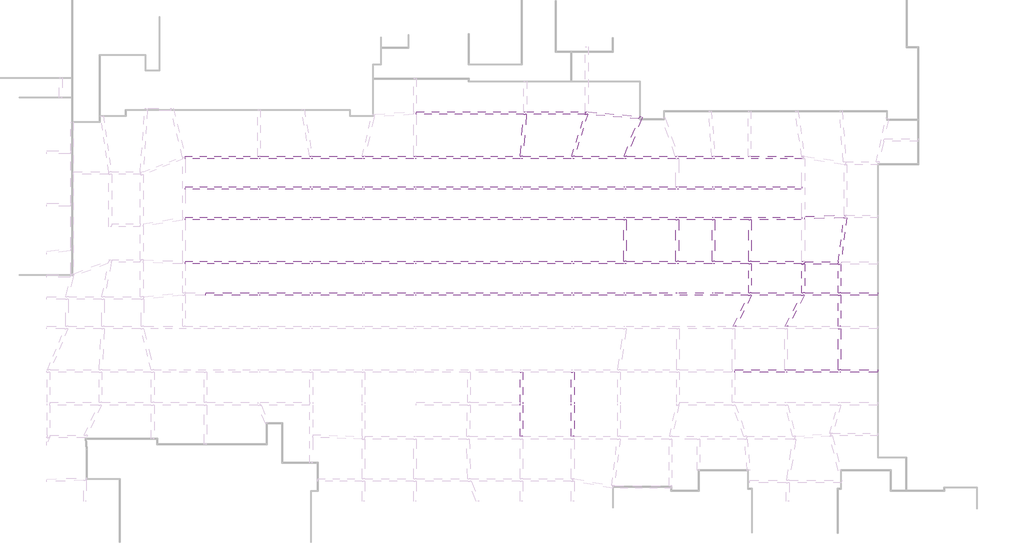
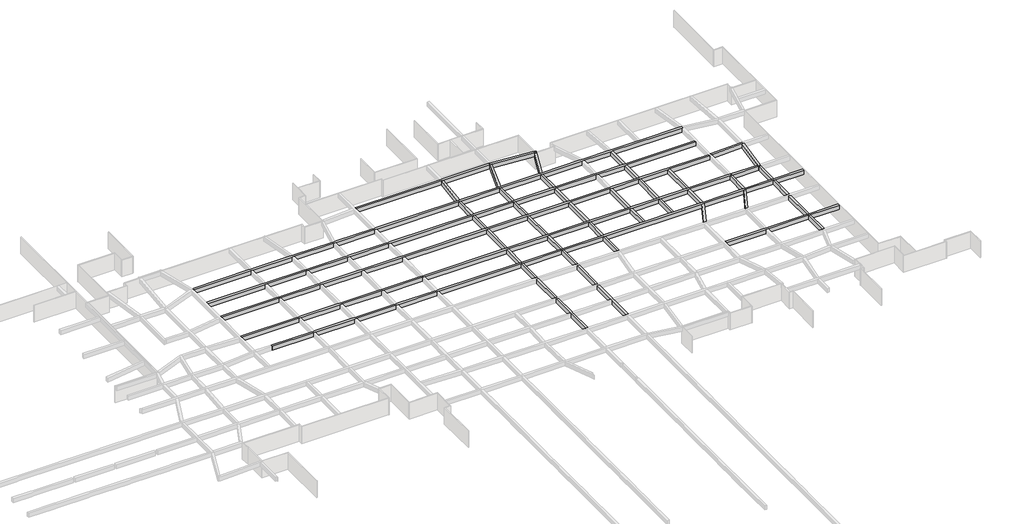
# One storey, part 44 of 45: 27 beams.
"""IFC4 building model written with IfcOpenShell, lengths in millimetres."""

from ifc_helpers import new_model, si_unit, frame, origin, place, context, project, spatial, polyline, outline, extrude, faceted_brep, element, save

model = new_model("IFC4")

# Units and contexts
model_context = context("Model", 3, world=origin())
ifc_project = project(units=[si_unit("LENGTHUNIT", "METRE", prefix="MILLI")], contexts=[model_context])

# Site, building, storey
site = spatial("IfcSite", under=ifc_project)
building = spatial("IfcBuilding", under=site)
storey = spatial("IfcBuildingStorey", under=building, Name="户型图", Elevation=0.0)

# Beams
placement = place(None, origin())
element("IfcBeam", 1, ObjectType="混凝土 - 矩形梁 : KL_beam", at=placement, inside=storey, context=model_context, shape_type="Brep", body=[
    faceted_brep([(63459.0283671, 163994.6607145, 3300.0), (63459.0283671, 163594.6607145, 3300.0), (63459.0283671, 163594.6607145, 2500.0), (63459.0283671, 163994.6607145, 2500.0), (57931.1254195, 163994.6607145, 3300.0), (57531.1254195, 163994.6607145, 3300.0), (52492.4652495, 163994.6607145, 3300.0), (52092.4652495, 163994.6607145, 3300.0), (44558.170888, 163994.6607145, 3300.0), (44158.170888, 163994.6607145, 3300.0), (39058.170888, 163994.6607145, 3300.0), (38658.170888, 163994.6607145, 3300.0), (33658.170888, 163994.6607145, 3300.0), (33258.170888, 163994.6607145, 3300.0), (25858.170888, 163994.6607145, 3300.0), (25458.170888, 163994.6607145, 3300.0), (18058.170888, 163994.6607145, 3300.0), (17658.170888, 163994.6607145, 3300.0), (10373.3027926, 163994.6607145, 3300.0), (9973.3027926, 163994.6607145, 3300.0), (-5504.3123934, 163994.6607145, 3300.0), (-5904.3123934, 163994.6607145, 3300.0), (-13220.6748317, 163994.6607145, 3300.0), (-13620.6748317, 163994.6607145, 3300.0), (-21020.6748317, 163994.6607145, 3300.0), (-21420.6748317, 163994.6607145, 3300.0), (-28820.6748317, 163994.6607145, 3300.0), (-29220.6748317, 163994.6607145, 3300.0), (-37009.4216094, 163994.6607145, 3300.0), (-37009.4216094, 163994.4687414, 3300.0), (-37009.4216094, 163594.6607145, 3300.0), (-29220.6748317, 163594.6607145, 3300.0), (-28820.6748317, 163594.6607145, 3300.0), (-21420.6748317, 163594.6607145, 3300.0), (-21020.6748317, 163594.6607145, 3300.0), (-13620.6748317, 163594.6607145, 3300.0), (-13220.6748317, 163594.6607145, 3300.0), (-5904.3123934, 163594.6607145, 3300.0), (-5504.3123934, 163594.6607145, 3300.0), (9973.3027926, 163594.6607145, 3300.0), (10373.3027926, 163594.6607145, 3300.0), (17658.170888, 163594.6607145, 3300.0), (18058.170888, 163594.6607145, 3300.0), (25458.170888, 163594.6607145, 3300.0), (25858.170888, 163594.6607145, 3300.0), (44084.7377305, 163594.6607145, 3300.0), (44529.7785067, 163594.6607145, 3300.0), (51966.0949121, 163594.6607145, 3300.0), (52415.0254072, 163594.6607145, 3300.0), (57531.1254195, 163594.6607145, 3300.0), (57931.1254195, 163594.6607145, 3300.0), (-37009.4216094, 163594.6607145, 2500.0), (-29220.6748317, 163594.6607145, 2500.0), (-28820.6748317, 163594.6607145, 2500.0), (-21420.6748317, 163594.6607145, 2500.0), (-21020.6748317, 163594.6607145, 2500.0), (-13620.6748317, 163594.6607145, 2500.0), (-13220.6748317, 163594.6607145, 2500.0), (-5904.3123934, 163594.6607145, 2500.0), (-5504.3123934, 163594.6607145, 2500.0), (9973.3027926, 163594.6607145, 2500.0), (10373.3027926, 163594.6607145, 2500.0), (17658.170888, 163594.6607145, 2500.0), (18058.170888, 163594.6607145, 2500.0), (25458.170888, 163594.6607145, 2500.0), (25858.170888, 163594.6607145, 2500.0), (44084.7377305, 163594.6607145, 2500.0), (44529.7785067, 163594.6607145, 2500.0), (51966.0949121, 163594.6607145, 2500.0), (52415.0254072, 163594.6607145, 2500.0), (57531.1254195, 163594.6607145, 2500.0), (57931.1254195, 163594.6607145, 2500.0), (-37009.4216094, 163994.4687414, 2500.0), (-37009.4216094, 163994.6607145, 2500.0), (-29220.6748317, 163994.6607145, 2500.0), (-28820.6748317, 163994.6607145, 2500.0), (-21420.6748317, 163994.6607145, 2500.0), (-21020.6748317, 163994.6607145, 2500.0), (-13620.6748317, 163994.6607145, 2500.0), (-13220.6748317, 163994.6607145, 2500.0), (-5904.3123934, 163994.6607145, 2500.0), (-5504.3123934, 163994.6607145, 2500.0), (9973.3027926, 163994.6607145, 2500.0), (10373.3027926, 163994.6607145, 2500.0), (17658.170888, 163994.6607145, 2500.0), (18058.170888, 163994.6607145, 2500.0), (25458.170888, 163994.6607145, 2500.0), (25858.170888, 163994.6607145, 2500.0), (33258.170888, 163994.6607145, 2500.0), (33658.170888, 163994.6607145, 2500.0), (38658.170888, 163994.6607145, 2500.0), (39058.170888, 163994.6607145, 2500.0), (44158.170888, 163994.6607145, 2500.0), (44558.170888, 163994.6607145, 2500.0), (52092.4652495, 163994.6607145, 2500.0), (52492.4652495, 163994.6607145, 2500.0), (57531.1254195, 163994.6607145, 2500.0), (57931.1254195, 163994.6607145, 2500.0)], [[[0, 1, 2, 3]], [[1, 0, 4, 5, 6, 7, 8, 9, 10, 11, 12, 13, 14, 15, 16, 17, 18, 19, 20, 21, 22, 23, 24, 25, 26, 27, 28, 29, 30, 31, 32, 33, 34, 35, 36, 37, 38, 39, 40, 41, 42, 43, 44, 45, 46, 47, 48, 49, 50]], [[2, 1, 50, 49, 48, 47, 46, 45, 44, 43, 42, 41, 40, 39, 38, 37, 36, 35, 34, 33, 32, 31, 30, 51, 52, 53, 54, 55, 56, 57, 58, 59, 60, 61, 62, 63, 64, 65, 66, 67, 68, 69, 70, 71]], [[3, 2, 71, 70, 69, 68, 67, 66, 65, 64, 63, 62, 61, 60, 59, 58, 57, 56, 55, 54, 53, 52, 51, 72, 73, 74, 75, 76, 77, 78, 79, 80, 81, 82, 83, 84, 85, 86, 87, 88, 89, 90, 91, 92, 93, 94, 95, 96, 97]], [[0, 3, 97, 96, 95, 94, 93, 92, 91, 90, 89, 88, 87, 86, 85, 84, 83, 82, 81, 80, 79, 78, 77, 76, 75, 74, 73, 28, 27, 26, 25, 24, 23, 22, 21, 20, 19, 18, 17, 16, 15, 14, 13, 12, 11, 10, 9, 8, 7, 6, 5, 4]], [[28, 73, 72, 51, 30, 29]]]),
])
element("IfcBeam", 2, ObjectType="混凝土 - 矩形梁 : KL_beam", at=placement, inside=storey, context=model_context, shape_type="Brep", body=[
    faceted_brep([(52292.9021454, 184394.3140025, 3300.0), (52048.8431015, 184394.3140025, 3300.0), (44458.170888, 184394.3140025, 3300.0), (44058.170888, 184394.3140025, 3300.0), (39044.6739052, 184394.3140025, 3300.0), (38643.697146, 184394.3140025, 3300.0), (33600.8295016, 184394.3140025, 3300.0), (33177.7812291, 184394.3140025, 3300.0), (25952.5239413, 184394.3140025, 3300.0), (25522.3855905, 184394.3140025, 3300.0), (18130.3080686, 184394.3140025, 3300.0), (17711.1861948, 184394.3140025, 3300.0), (10391.598587, 184394.3140025, 3300.0), (9990.070652, 184394.3140025, 3300.0), (-5504.3123934, 184394.3140025, 3300.0), (-5904.3123934, 184394.3140025, 3300.0), (-13169.2403719, 184394.3140025, 3300.0), (-13579.762015, 184394.3140025, 3300.0), (-21052.8549054, 184394.3140025, 3300.0), (-21459.0255502, 184394.3140025, 3300.0), (-28820.6748317, 184394.3140025, 3300.0), (-29220.6748317, 184394.3140025, 3300.0), (-40064.3312613, 184394.3140025, 3300.0), (-40020.6748317, 184219.2176267, 3300.0), (-40020.6748317, 183994.3140025, 3300.0), (-29220.6748317, 183994.3140025, 3300.0), (-28820.6748317, 183994.3140025, 3300.0), (-21420.6748317, 183994.3140025, 3300.0), (-21020.6748317, 183994.3140025, 3300.0), (-13620.6748317, 183994.3140025, 3300.0), (-13220.6748317, 183994.3140025, 3300.0), (-5904.3123934, 183994.3140025, 3300.0), (-5504.3123934, 183994.3140025, 3300.0), (9973.3027926, 183994.3140025, 3300.0), (10373.3027926, 183994.3140025, 3300.0), (17658.170888, 183994.3140025, 3300.0), (18058.170888, 183994.3140025, 3300.0), (25458.170888, 183994.3140025, 3300.0), (25858.170888, 183994.3140025, 3300.0), (33258.170888, 183994.3140025, 3300.0), (33658.170888, 183994.3140025, 3300.0), (38658.170888, 183994.3140025, 3300.0), (39058.170888, 183994.3140025, 3300.0), (52092.6053307, 183994.3140025, 3300.0), (52264.9314206, 183994.3140025, 3300.0), (52264.9314206, 183994.3140025, 2500.0), (-40020.6748317, 183994.3140025, 2500.0), (-29220.6748317, 183994.3140025, 2500.0), (-28820.6748317, 183994.3140025, 2500.0), (-21420.6748317, 183994.3140025, 2500.0), (-21020.6748317, 183994.3140025, 2500.0), (-13620.6748317, 183994.3140025, 2500.0), (-13220.6748317, 183994.3140025, 2500.0), (-5904.3123934, 183994.3140025, 2500.0), (-5504.3123934, 183994.3140025, 2500.0), (9973.3027926, 183994.3140025, 2500.0), (10373.3027926, 183994.3140025, 2500.0), (17658.170888, 183994.3140025, 2500.0), (18058.170888, 183994.3140025, 2500.0), (25458.170888, 183994.3140025, 2500.0), (25858.170888, 183994.3140025, 2500.0), (33258.170888, 183994.3140025, 2500.0), (33658.170888, 183994.3140025, 2500.0), (38658.170888, 183994.3140025, 2500.0), (39058.170888, 183994.3140025, 2500.0), (52092.6053307, 183994.3140025, 2500.0), (-40064.3312613, 184394.3140025, 2500.0), (-29220.6748317, 184394.3140025, 2500.0), (-28820.6748317, 184394.3140025, 2500.0), (-21459.0255502, 184394.3140025, 2500.0), (-21052.8549054, 184394.3140025, 2500.0), (-13579.762015, 184394.3140025, 2500.0), (-13169.2403719, 184394.3140025, 2500.0), (-5904.3123934, 184394.3140025, 2500.0), (-5504.3123934, 184394.3140025, 2500.0), (9990.070652, 184394.3140025, 2500.0), (10391.598587, 184394.3140025, 2500.0), (17711.1861948, 184394.3140025, 2500.0), (18130.3080686, 184394.3140025, 2500.0), (25522.3855905, 184394.3140025, 2500.0), (25952.5239413, 184394.3140025, 2500.0), (33177.7812291, 184394.3140025, 2500.0), (33600.8295016, 184394.3140025, 2500.0), (38643.697146, 184394.3140025, 2500.0), (39044.6739052, 184394.3140025, 2500.0), (44058.170888, 184394.3140025, 2500.0), (44458.170888, 184394.3140025, 2500.0), (52048.8431015, 184394.3140025, 2500.0), (52292.9021454, 184394.3140025, 2500.0), (-40020.6748317, 184219.2176267, 2500.0)], [[[0, 1, 2, 3, 4, 5, 6, 7, 8, 9, 10, 11, 12, 13, 14, 15, 16, 17, 18, 19, 20, 21, 22, 23, 24, 25, 26, 27, 28, 29, 30, 31, 32, 33, 34, 35, 36, 37, 38, 39, 40, 41, 42, 43, 44]], [[45, 44, 43, 42, 41, 40, 39, 38, 37, 36, 35, 34, 33, 32, 31, 30, 29, 28, 27, 26, 25, 24, 46, 47, 48, 49, 50, 51, 52, 53, 54, 55, 56, 57, 58, 59, 60, 61, 62, 63, 64, 65]], [[66, 67, 68, 69, 70, 71, 72, 73, 74, 75, 76, 77, 78, 79, 80, 81, 82, 83, 84, 85, 86, 87, 88, 45, 65, 64, 63, 62, 61, 60, 59, 58, 57, 56, 55, 54, 53, 52, 51, 50, 49, 48, 47, 46, 89]], [[22, 21, 20, 19, 18, 17, 16, 15, 14, 13, 12, 11, 10, 9, 8, 7, 6, 5, 4, 3, 2, 1, 0, 88, 87, 86, 85, 84, 83, 82, 81, 80, 79, 78, 77, 76, 75, 74, 73, 72, 71, 70, 69, 68, 67, 66]], [[89, 23, 22, 66]], [[23, 89, 46, 24]], [[0, 44, 45, 88]]]),
])
element("IfcBeam", 3, ObjectType="混凝土 - 矩形梁 : KL_beam", at=placement, inside=storey, context=model_context, shape_type="Brep", body=[
    faceted_brep([(-40020.6748317, 179811.4368869, 3300.0), (-40020.6748317, 179411.4368869, 3300.0), (-29220.6748317, 179411.4368869, 3300.0), (-28820.6748317, 179411.4368869, 3300.0), (-21420.6748317, 179411.4368869, 3300.0), (-21020.6748317, 179411.4368869, 3300.0), (-13620.6748317, 179411.4368869, 3300.0), (-13220.6748317, 179411.4368869, 3300.0), (-5904.3123934, 179411.4368869, 3300.0), (-5504.3123934, 179411.4368869, 3300.0), (9973.3027926, 179411.4368869, 3300.0), (10373.3027926, 179411.4368869, 3300.0), (17658.170888, 179411.4368869, 3300.0), (18058.170888, 179411.4368869, 3300.0), (25458.170888, 179411.4368869, 3300.0), (25858.170888, 179411.4368869, 3300.0), (33258.170888, 179411.4368869, 3300.0), (33658.170888, 179411.4368869, 3300.0), (38658.170888, 179411.4368869, 3300.0), (39058.170888, 179411.4368869, 3300.0), (52092.6053307, 179411.4368869, 3300.0), (52092.6053307, 179811.4368869, 3300.0), (39058.170888, 179811.4368869, 3300.0), (38658.170888, 179811.4368869, 3300.0), (33658.170888, 179811.4368869, 3300.0), (33258.170888, 179811.4368869, 3300.0), (25858.170888, 179811.4368869, 3300.0), (25458.170888, 179811.4368869, 3300.0), (18058.170888, 179811.4368869, 3300.0), (17658.170888, 179811.4368869, 3300.0), (10373.3027926, 179811.4368869, 3300.0), (9973.3027926, 179811.4368869, 3300.0), (-5504.3123934, 179811.4368869, 3300.0), (-5904.3123934, 179811.4368869, 3300.0), (-13220.6748317, 179811.4368869, 3300.0), (-13620.6748317, 179811.4368869, 3300.0), (-21020.6748317, 179811.4368869, 3300.0), (-21420.6748317, 179811.4368869, 3300.0), (-28820.6748317, 179811.4368869, 3300.0), (-29220.6748317, 179811.4368869, 3300.0), (-40020.6748317, 179811.4368869, 2500.0), (52092.6053307, 179811.4368869, 2500.0), (39058.170888, 179811.4368869, 2500.0), (38658.170888, 179811.4368869, 2500.0), (33658.170888, 179811.4368869, 2500.0), (33258.170888, 179811.4368869, 2500.0), (25858.170888, 179811.4368869, 2500.0), (25458.170888, 179811.4368869, 2500.0), (18058.170888, 179811.4368869, 2500.0), (17658.170888, 179811.4368869, 2500.0), (10373.3027926, 179811.4368869, 2500.0), (9973.3027926, 179811.4368869, 2500.0), (-5504.3123934, 179811.4368869, 2500.0), (-5904.3123934, 179811.4368869, 2500.0), (-13220.6748317, 179811.4368869, 2500.0), (-13620.6748317, 179811.4368869, 2500.0), (-21020.6748317, 179811.4368869, 2500.0), (-21420.6748317, 179811.4368869, 2500.0), (-28820.6748317, 179811.4368869, 2500.0), (-29220.6748317, 179811.4368869, 2500.0), (-40020.6748317, 179411.4368869, 2500.0), (52092.6053307, 179411.4368869, 2500.0), (39058.170888, 179411.4368869, 2500.0), (38658.170888, 179411.4368869, 2500.0), (33658.170888, 179411.4368869, 2500.0), (33258.170888, 179411.4368869, 2500.0), (25858.170888, 179411.4368869, 2500.0), (25458.170888, 179411.4368869, 2500.0), (18058.170888, 179411.4368869, 2500.0), (17658.170888, 179411.4368869, 2500.0), (10373.3027926, 179411.4368869, 2500.0), (9973.3027926, 179411.4368869, 2500.0), (-5504.3123934, 179411.4368869, 2500.0), (-5904.3123934, 179411.4368869, 2500.0), (-13220.6748317, 179411.4368869, 2500.0), (-13620.6748317, 179411.4368869, 2500.0), (-21020.6748317, 179411.4368869, 2500.0), (-21420.6748317, 179411.4368869, 2500.0), (-28820.6748317, 179411.4368869, 2500.0), (-29220.6748317, 179411.4368869, 2500.0)], [[[0, 1, 2, 3, 4, 5, 6, 7, 8, 9, 10, 11, 12, 13, 14, 15, 16, 17, 18, 19, 20, 21, 22, 23, 24, 25, 26, 27, 28, 29, 30, 31, 32, 33, 34, 35, 36, 37, 38, 39]], [[40, 0, 39, 38, 37, 36, 35, 34, 33, 32, 31, 30, 29, 28, 27, 26, 25, 24, 23, 22, 21, 41, 42, 43, 44, 45, 46, 47, 48, 49, 50, 51, 52, 53, 54, 55, 56, 57, 58, 59]], [[60, 40, 59, 58, 57, 56, 55, 54, 53, 52, 51, 50, 49, 48, 47, 46, 45, 44, 43, 42, 41, 61, 62, 63, 64, 65, 66, 67, 68, 69, 70, 71, 72, 73, 74, 75, 76, 77, 78, 79]], [[1, 60, 79, 78, 77, 76, 75, 74, 73, 72, 71, 70, 69, 68, 67, 66, 65, 64, 63, 62, 61, 20, 19, 18, 17, 16, 15, 14, 13, 12, 11, 10, 9, 8, 7, 6, 5, 4, 3, 2]], [[1, 0, 40, 60]], [[21, 20, 61, 41]]]),
])
element("IfcBeam", 4, ObjectType="混凝土 - 矩形梁 : KL_beam", at=placement, inside=storey, context=model_context, shape_type="Brep", body=[
    faceted_brep([(-40020.6748317, 175259.2955299, 3300.0), (-40020.6748317, 174859.2955299, 3300.0), (-29220.6748317, 174859.2955299, 3300.0), (-28820.6748317, 174859.2955299, 3300.0), (-21420.6748317, 174859.2955299, 3300.0), (-21020.6748317, 174859.2955299, 3300.0), (-13620.6748317, 174859.2955299, 3300.0), (-13220.6748317, 174859.2955299, 3300.0), (-5904.3123934, 174859.2955299, 3300.0), (-5504.3123934, 174859.2955299, 3300.0), (9973.3027926, 174859.2955299, 3300.0), (10373.3027926, 174859.2955299, 3300.0), (17658.170888, 174859.2955299, 3300.0), (18058.170888, 174859.2955299, 3300.0), (25458.170888, 174859.2955299, 3300.0), (25858.170888, 174859.2955299, 3300.0), (33258.170888, 174859.2955299, 3300.0), (33658.170888, 174859.2955299, 3300.0), (38658.170888, 174859.2955299, 3300.0), (39058.170888, 174859.2955299, 3300.0), (44158.170888, 174859.2955299, 3300.0), (44558.170888, 174859.2955299, 3300.0), (52092.6053307, 174859.2955299, 3300.0), (52092.6053307, 175259.2955299, 3300.0), (39058.170888, 175259.2955299, 3300.0), (38658.170888, 175259.2955299, 3300.0), (33658.170888, 175259.2955299, 3300.0), (33258.170888, 175259.2955299, 3300.0), (25858.170888, 175259.2955299, 3300.0), (25458.170888, 175259.2955299, 3300.0), (18058.170888, 175259.2955299, 3300.0), (17658.170888, 175259.2955299, 3300.0), (10373.3027926, 175259.2955299, 3300.0), (9973.3027926, 175259.2955299, 3300.0), (-5504.3123934, 175259.2955299, 3300.0), (-5904.3123934, 175259.2955299, 3300.0), (-13220.6748317, 175259.2955299, 3300.0), (-13620.6748317, 175259.2955299, 3300.0), (-21020.6748317, 175259.2955299, 3300.0), (-21420.6748317, 175259.2955299, 3300.0), (-28820.6748317, 175259.2955299, 3300.0), (-29220.6748317, 175259.2955299, 3300.0), (-40020.6748317, 174859.2955299, 2500.0), (-29220.6748317, 174859.2955299, 2500.0), (-28820.6748317, 174859.2955299, 2500.0), (-21420.6748317, 174859.2955299, 2500.0), (-21020.6748317, 174859.2955299, 2500.0), (-13620.6748317, 174859.2955299, 2500.0), (-13220.6748317, 174859.2955299, 2500.0), (-5904.3123934, 174859.2955299, 2500.0), (-5504.3123934, 174859.2955299, 2500.0), (9973.3027926, 174859.2955299, 2500.0), (10373.3027926, 174859.2955299, 2500.0), (17658.170888, 174859.2955299, 2500.0), (18058.170888, 174859.2955299, 2500.0), (25458.170888, 174859.2955299, 2500.0), (25858.170888, 174859.2955299, 2500.0), (33258.170888, 174859.2955299, 2500.0), (33658.170888, 174859.2955299, 2500.0), (38658.170888, 174859.2955299, 2500.0), (39058.170888, 174859.2955299, 2500.0), (44158.170888, 174859.2955299, 2500.0), (44558.170888, 174859.2955299, 2500.0), (52092.6053307, 174859.2955299, 2500.0), (-40020.6748317, 175259.2955299, 2500.0), (-29220.6748317, 175259.2955299, 2500.0), (-28820.6748317, 175259.2955299, 2500.0), (-21420.6748317, 175259.2955299, 2500.0), (-21020.6748317, 175259.2955299, 2500.0), (-13620.6748317, 175259.2955299, 2500.0), (-13220.6748317, 175259.2955299, 2500.0), (-5904.3123934, 175259.2955299, 2500.0), (-5504.3123934, 175259.2955299, 2500.0), (9973.3027926, 175259.2955299, 2500.0), (10373.3027926, 175259.2955299, 2500.0), (17658.170888, 175259.2955299, 2500.0), (18058.170888, 175259.2955299, 2500.0), (25458.170888, 175259.2955299, 2500.0), (25858.170888, 175259.2955299, 2500.0), (33258.170888, 175259.2955299, 2500.0), (33658.170888, 175259.2955299, 2500.0), (38658.170888, 175259.2955299, 2500.0), (39058.170888, 175259.2955299, 2500.0), (52092.6053307, 175259.2955299, 2500.0)], [[[0, 1, 2, 3, 4, 5, 6, 7, 8, 9, 10, 11, 12, 13, 14, 15, 16, 17, 18, 19, 20, 21, 22, 23, 24, 25, 26, 27, 28, 29, 30, 31, 32, 33, 34, 35, 36, 37, 38, 39, 40, 41]], [[1, 42, 43, 44, 45, 46, 47, 48, 49, 50, 51, 52, 53, 54, 55, 56, 57, 58, 59, 60, 61, 62, 63, 22, 21, 20, 19, 18, 17, 16, 15, 14, 13, 12, 11, 10, 9, 8, 7, 6, 5, 4, 3, 2]], [[42, 64, 65, 66, 67, 68, 69, 70, 71, 72, 73, 74, 75, 76, 77, 78, 79, 80, 81, 82, 83, 63, 62, 61, 60, 59, 58, 57, 56, 55, 54, 53, 52, 51, 50, 49, 48, 47, 46, 45, 44, 43]], [[64, 0, 41, 40, 39, 38, 37, 36, 35, 34, 33, 32, 31, 30, 29, 28, 27, 26, 25, 24, 23, 83, 82, 81, 80, 79, 78, 77, 76, 75, 74, 73, 72, 71, 70, 69, 68, 67, 66, 65]], [[1, 0, 64, 42]], [[23, 22, 63, 83]]]),
])
element("IfcBeam", 5, ObjectType="混凝土 - 矩形梁 : KL_beam", at=placement, inside=storey, context=model_context, shape_type="Brep", body=[
    faceted_brep([(52492.6053307, 168316.2365071, 3300.0), (52492.6053307, 168641.1854865, 3300.0), (52492.6053307, 168716.2365071, 3300.0), (52092.6053307, 168716.2365071, 3300.0), (44558.170888, 168716.2365071, 3300.0), (44158.170888, 168716.2365071, 3300.0), (39058.170888, 168716.2365071, 3300.0), (38658.170888, 168716.2365071, 3300.0), (33658.170888, 168716.2365071, 3300.0), (33258.170888, 168716.2365071, 3300.0), (25858.170888, 168716.2365071, 3300.0), (25458.170888, 168716.2365071, 3300.0), (18058.170888, 168716.2365071, 3300.0), (17658.170888, 168716.2365071, 3300.0), (10373.3027926, 168716.2365071, 3300.0), (9973.3027926, 168716.2365071, 3300.0), (-5504.3123934, 168716.2365071, 3300.0), (-5904.3123934, 168716.2365071, 3300.0), (-13220.6748317, 168716.2365071, 3300.0), (-13620.6748317, 168716.2365071, 3300.0), (-21020.6748317, 168716.2365071, 3300.0), (-21420.6748317, 168716.2365071, 3300.0), (-28820.6748317, 168716.2365071, 3300.0), (-29220.6748317, 168716.2365071, 3300.0), (-40020.6748317, 168716.2365071, 3300.0), (-40020.6748317, 168316.2365071, 3300.0), (-29220.6748317, 168316.2365071, 3300.0), (-28820.6748317, 168316.2365071, 3300.0), (-21420.6748317, 168316.2365071, 3300.0), (-21020.6748317, 168316.2365071, 3300.0), (-13620.6748317, 168316.2365071, 3300.0), (-13220.6748317, 168316.2365071, 3300.0), (-5904.3123934, 168316.2365071, 3300.0), (-5504.3123934, 168316.2365071, 3300.0), (9973.3027926, 168316.2365071, 3300.0), (10373.3027926, 168316.2365071, 3300.0), (17658.170888, 168316.2365071, 3300.0), (18058.170888, 168316.2365071, 3300.0), (25458.170888, 168316.2365071, 3300.0), (25858.170888, 168316.2365071, 3300.0), (33258.170888, 168316.2365071, 3300.0), (33658.170888, 168316.2365071, 3300.0), (38658.170888, 168316.2365071, 3300.0), (39058.170888, 168316.2365071, 3300.0), (44158.170888, 168316.2365071, 3300.0), (44558.170888, 168316.2365071, 3300.0), (52092.4652495, 168316.2365071, 3300.0), (52492.6053307, 168716.2365071, 2500.0), (52092.6053307, 168716.2365071, 2500.0), (44558.170888, 168716.2365071, 2500.0), (44158.170888, 168716.2365071, 2500.0), (39058.170888, 168716.2365071, 2500.0), (38658.170888, 168716.2365071, 2500.0), (33658.170888, 168716.2365071, 2500.0), (33258.170888, 168716.2365071, 2500.0), (25858.170888, 168716.2365071, 2500.0), (25458.170888, 168716.2365071, 2500.0), (18058.170888, 168716.2365071, 2500.0), (17658.170888, 168716.2365071, 2500.0), (10373.3027926, 168716.2365071, 2500.0), (9973.3027926, 168716.2365071, 2500.0), (-5504.3123934, 168716.2365071, 2500.0), (-5904.3123934, 168716.2365071, 2500.0), (-13220.6748317, 168716.2365071, 2500.0), (-13620.6748317, 168716.2365071, 2500.0), (-21020.6748317, 168716.2365071, 2500.0), (-21420.6748317, 168716.2365071, 2500.0), (-28820.6748317, 168716.2365071, 2500.0), (-29220.6748317, 168716.2365071, 2500.0), (-40020.6748317, 168716.2365071, 2500.0), (52492.6053307, 168641.1854865, 2500.0), (52492.6053307, 168316.2365071, 2500.0), (52092.4652495, 168316.2365071, 2500.0), (44558.170888, 168316.2365071, 2500.0), (44158.170888, 168316.2365071, 2500.0), (39058.170888, 168316.2365071, 2500.0), (38658.170888, 168316.2365071, 2500.0), (33658.170888, 168316.2365071, 2500.0), (33258.170888, 168316.2365071, 2500.0), (25858.170888, 168316.2365071, 2500.0), (25458.170888, 168316.2365071, 2500.0), (18058.170888, 168316.2365071, 2500.0), (17658.170888, 168316.2365071, 2500.0), (10373.3027926, 168316.2365071, 2500.0), (9973.3027926, 168316.2365071, 2500.0), (-5504.3123934, 168316.2365071, 2500.0), (-5904.3123934, 168316.2365071, 2500.0), (-13220.6748317, 168316.2365071, 2500.0), (-13620.6748317, 168316.2365071, 2500.0), (-21020.6748317, 168316.2365071, 2500.0), (-21420.6748317, 168316.2365071, 2500.0), (-28820.6748317, 168316.2365071, 2500.0), (-29220.6748317, 168316.2365071, 2500.0), (-40020.6748317, 168316.2365071, 2500.0)], [[[0, 1, 2, 3, 4, 5, 6, 7, 8, 9, 10, 11, 12, 13, 14, 15, 16, 17, 18, 19, 20, 21, 22, 23, 24, 25, 26, 27, 28, 29, 30, 31, 32, 33, 34, 35, 36, 37, 38, 39, 40, 41, 42, 43, 44, 45, 46]], [[2, 47, 48, 49, 50, 51, 52, 53, 54, 55, 56, 57, 58, 59, 60, 61, 62, 63, 64, 65, 66, 67, 68, 69, 24, 23, 22, 21, 20, 19, 18, 17, 16, 15, 14, 13, 12, 11, 10, 9, 8, 7, 6, 5, 4, 3]], [[47, 70, 71, 72, 73, 74, 75, 76, 77, 78, 79, 80, 81, 82, 83, 84, 85, 86, 87, 88, 89, 90, 91, 92, 93, 69, 68, 67, 66, 65, 64, 63, 62, 61, 60, 59, 58, 57, 56, 55, 54, 53, 52, 51, 50, 49, 48]], [[71, 0, 46, 45, 44, 43, 42, 41, 40, 39, 38, 37, 36, 35, 34, 33, 32, 31, 30, 29, 28, 27, 26, 25, 93, 92, 91, 90, 89, 88, 87, 86, 85, 84, 83, 82, 81, 80, 79, 78, 77, 76, 75, 74, 73, 72]], [[25, 24, 69, 93]], [[2, 1, 0, 71, 70, 47]]]),
])
element("IfcBeam", 6, ObjectType="混凝土 - 矩形梁 : KL_beam", at=placement, inside=storey, context=model_context, shape_type="SweptSolid", body=[
    extrude(outline(polyline([(10535.9846193, 190634.1392013), (10937.5125543, 190634.1392013), (10391.598587, 184394.3140025), (9990.070652, 184394.3140025), (10535.9846193, 190634.1392013)])), frame((0.0, 0.0, 2500.0), z_axis=(0.0, 0.0, 1.0), x_axis=(1.0, 0.0, 0.0)), (0.0, 0.0, 1.0), 800.0),
])
element("IfcBeam", 7, ObjectType="混凝土 - 矩形梁 : KL_beam", at=placement, inside=storey, context=model_context, shape_type="Brep", body=[
    faceted_brep([(10373.3027926, 183994.3140025, 3300.0), (9973.3027926, 183994.3140025, 3300.0), (9973.3027926, 179811.4368869, 3300.0), (10373.3027926, 179811.4368869, 3300.0), (9973.3027926, 183994.3140025, 2500.0), (9973.3027926, 179811.4368869, 2500.0), (10373.3027926, 183994.3140025, 2500.0), (10373.3027926, 179811.4368869, 2500.0)], [[[0, 1, 2, 3]], [[1, 4, 5, 2]], [[4, 6, 7, 5]], [[6, 0, 3, 7]], [[1, 0, 6, 4]], [[3, 2, 5, 7]]]),
    faceted_brep([(9973.3027926, 152079.7935386, 3300.0), (10373.3027926, 152079.7935386, 3300.0), (10373.3027926, 152079.7935386, 2500.0), (9973.3027926, 152079.7935386, 2500.0), (9973.3027926, 147579.5060773, 3300.0), (9973.3027926, 147179.5060773, 3300.0), (9973.3027926, 142504.5723204, 3300.0), (10373.3027926, 142504.5723204, 3300.0), (10373.3027926, 147179.5060773, 3300.0), (10373.3027926, 147579.5060773, 3300.0), (9973.3027926, 147579.5060773, 2500.0), (9973.3027926, 147179.5060773, 2500.0), (9973.3027926, 142504.5723204, 2500.0), (10373.3027926, 147579.5060773, 2500.0), (10373.3027926, 147179.5060773, 2500.0), (10373.3027926, 142504.5723204, 2500.0)], [[[0, 1, 2, 3]], [[1, 0, 4, 5, 6, 7, 8, 9]], [[0, 3, 10, 11, 12, 6, 5, 4]], [[3, 2, 13, 14, 15, 12, 11, 10]], [[2, 1, 9, 8, 7, 15, 14, 13]], [[7, 6, 12, 15]]]),
    faceted_brep([(10373.3027926, 152479.7935386, 3300.0), (9973.3027926, 152479.7935386, 3300.0), (9973.3027926, 152479.7935386, 2500.0), (10373.3027926, 152479.7935386, 2500.0), (9973.3027926, 158578.3181414, 3300.0), (10373.3027926, 158578.3181414, 3300.0), (10373.3027926, 158578.3181414, 2500.0), (9973.3027926, 158578.3181414, 2500.0)], [[[0, 1, 2, 3]], [[4, 5, 6, 7]], [[1, 0, 5, 4]], [[2, 1, 4, 7]], [[3, 2, 7, 6]], [[0, 3, 6, 5]]]),
    faceted_brep([(10373.3027926, 158978.3181414, 3300.0), (9973.3027926, 158978.3181414, 3300.0), (9973.3027926, 158978.3181414, 2500.0), (10373.3027926, 158978.3181414, 2500.0), (9973.3027926, 163594.6607145, 3300.0), (10373.3027926, 163594.6607145, 3300.0), (10373.3027926, 163594.6607145, 2500.0), (9973.3027926, 163594.6607145, 2500.0)], [[[0, 1, 2, 3]], [[4, 5, 6, 7]], [[1, 0, 5, 4]], [[2, 1, 4, 7]], [[3, 2, 7, 6]], [[0, 3, 6, 5]]]),
    faceted_brep([(10373.3027926, 163994.6607145, 3300.0), (9973.3027926, 163994.6607145, 3300.0), (9973.3027926, 163994.6607145, 2500.0), (10373.3027926, 163994.6607145, 2500.0), (9973.3027926, 168316.2365071, 3300.0), (10373.3027926, 168316.2365071, 3300.0), (10373.3027926, 168316.2365071, 2500.0), (9973.3027926, 168316.2365071, 2500.0)], [[[0, 1, 2, 3]], [[4, 5, 6, 7]], [[1, 0, 5, 4]], [[2, 1, 4, 7]], [[3, 2, 7, 6]], [[0, 3, 6, 5]]]),
    faceted_brep([(9973.3027926, 179411.4368869, 3300.0), (10373.3027926, 179411.4368869, 3300.0), (10373.3027926, 179411.4368869, 2500.0), (9973.3027926, 179411.4368869, 2500.0), (10373.3027926, 175259.2955299, 3300.0), (9973.3027926, 175259.2955299, 3300.0), (9973.3027926, 175259.2955299, 2500.0), (10373.3027926, 175259.2955299, 2500.0)], [[[0, 1, 2, 3]], [[4, 5, 6, 7]], [[1, 0, 5, 4]], [[0, 3, 6, 5]], [[3, 2, 7, 6]], [[2, 1, 4, 7]]]),
    faceted_brep([(9973.3027926, 174859.2955299, 3300.0), (10373.3027926, 174859.2955299, 3300.0), (10373.3027926, 174859.2955299, 2500.0), (9973.3027926, 174859.2955299, 2500.0), (10373.3027926, 168716.2365071, 3300.0), (9973.3027926, 168716.2365071, 3300.0), (9973.3027926, 168716.2365071, 2500.0), (10373.3027926, 168716.2365071, 2500.0)], [[[0, 1, 2, 3]], [[4, 5, 6, 7]], [[1, 0, 5, 4]], [[0, 3, 6, 5]], [[3, 2, 7, 6]], [[2, 1, 4, 7]]]),
])
element("IfcBeam", 8, ObjectType="混凝土 - 矩形梁 : KL_beam", at=placement, inside=storey, context=model_context, shape_type="Brep", body=[
    faceted_brep([(18058.170888, 183994.3140025, 3300.0), (17658.170888, 183994.3140025, 3300.0), (17658.170888, 179811.4368869, 3300.0), (18058.170888, 179811.4368869, 3300.0), (17658.170888, 183994.3140025, 2500.0), (17658.170888, 179811.4368869, 2500.0), (18058.170888, 183994.3140025, 2500.0), (18058.170888, 179811.4368869, 2500.0)], [[[0, 1, 2, 3]], [[1, 4, 5, 2]], [[4, 6, 7, 5]], [[6, 0, 3, 7]], [[1, 0, 6, 4]], [[3, 2, 5, 7]]]),
    faceted_brep([(17658.170888, 152079.7935386, 3300.0), (18058.170888, 152079.7935386, 3300.0), (18058.170888, 152079.7935386, 2500.0), (17658.170888, 152079.7935386, 2500.0), (17658.170888, 147579.5060773, 3300.0), (17658.170888, 147179.5060773, 3300.0), (17658.170888, 142504.5723204, 3300.0), (18058.170888, 142504.5723204, 3300.0), (18058.170888, 147179.5060773, 3300.0), (18058.170888, 147579.5060773, 3300.0), (17658.170888, 147579.5060773, 2500.0), (17658.170888, 147179.5060773, 2500.0), (17658.170888, 142504.5723204, 2500.0), (18058.170888, 147579.5060773, 2500.0), (18058.170888, 147179.5060773, 2500.0), (18058.170888, 142504.5723204, 2500.0)], [[[0, 1, 2, 3]], [[1, 0, 4, 5, 6, 7, 8, 9]], [[0, 3, 10, 11, 12, 6, 5, 4]], [[3, 2, 13, 14, 15, 12, 11, 10]], [[2, 1, 9, 8, 7, 15, 14, 13]], [[7, 6, 12, 15]]]),
    faceted_brep([(18058.170888, 152479.7935386, 3300.0), (17658.170888, 152479.7935386, 3300.0), (17658.170888, 152479.7935386, 2500.0), (18058.170888, 152479.7935386, 2500.0), (17658.170888, 158578.3181414, 3300.0), (18058.170888, 158578.3181414, 3300.0), (18058.170888, 158578.3181414, 2500.0), (17658.170888, 158578.3181414, 2500.0)], [[[0, 1, 2, 3]], [[4, 5, 6, 7]], [[1, 0, 5, 4]], [[2, 1, 4, 7]], [[3, 2, 7, 6]], [[0, 3, 6, 5]]]),
    faceted_brep([(18058.170888, 158978.3181414, 3300.0), (17658.170888, 158978.3181414, 3300.0), (17658.170888, 158978.3181414, 2500.0), (18058.170888, 158978.3181414, 2500.0), (17658.170888, 163594.6607145, 3300.0), (18058.170888, 163594.6607145, 3300.0), (18058.170888, 163594.6607145, 2500.0), (17658.170888, 163594.6607145, 2500.0)], [[[0, 1, 2, 3]], [[4, 5, 6, 7]], [[1, 0, 5, 4]], [[2, 1, 4, 7]], [[3, 2, 7, 6]], [[0, 3, 6, 5]]]),
    faceted_brep([(18058.170888, 163994.6607145, 3300.0), (17658.170888, 163994.6607145, 3300.0), (17658.170888, 163994.6607145, 2500.0), (18058.170888, 163994.6607145, 2500.0), (17658.170888, 168316.2365071, 3300.0), (18058.170888, 168316.2365071, 3300.0), (18058.170888, 168316.2365071, 2500.0), (17658.170888, 168316.2365071, 2500.0)], [[[0, 1, 2, 3]], [[4, 5, 6, 7]], [[1, 0, 5, 4]], [[2, 1, 4, 7]], [[3, 2, 7, 6]], [[0, 3, 6, 5]]]),
    faceted_brep([(17658.170888, 179411.4368869, 3300.0), (18058.170888, 179411.4368869, 3300.0), (18058.170888, 179411.4368869, 2500.0), (17658.170888, 179411.4368869, 2500.0), (18058.170888, 175259.2955299, 3300.0), (17658.170888, 175259.2955299, 3300.0), (17658.170888, 175259.2955299, 2500.0), (18058.170888, 175259.2955299, 2500.0)], [[[0, 1, 2, 3]], [[4, 5, 6, 7]], [[1, 0, 5, 4]], [[0, 3, 6, 5]], [[3, 2, 7, 6]], [[2, 1, 4, 7]]]),
    faceted_brep([(17658.170888, 174859.2955299, 3300.0), (18058.170888, 174859.2955299, 3300.0), (18058.170888, 174859.2955299, 2500.0), (17658.170888, 174859.2955299, 2500.0), (18058.170888, 168716.2365071, 3300.0), (17658.170888, 168716.2365071, 3300.0), (17658.170888, 168716.2365071, 2500.0), (18058.170888, 168716.2365071, 2500.0)], [[[0, 1, 2, 3]], [[4, 5, 6, 7]], [[1, 0, 5, 4]], [[0, 3, 6, 5]], [[3, 2, 7, 6]], [[2, 1, 4, 7]]]),
])
element("IfcBeam", 9, ObjectType="混凝土 - 矩形梁 : KL_beam", at=placement, inside=storey, context=model_context, shape_type="SweptSolid", body=[
    extrude(outline(polyline([(25458.170888, 183994.3140025), (25858.170888, 183994.3140025), (25858.170888, 179811.4368869), (25458.170888, 179811.4368869), (25458.170888, 183994.3140025)])), frame((0.0, 0.0, 2500.0), z_axis=(0.0, 0.0, 1.0), x_axis=(1.0, 0.0, 0.0)), (0.0, 0.0, 1.0), 800.0),
    extrude(outline(polyline([(25858.170888, 158978.3181414), (25458.170888, 158978.3181414), (25458.170888, 163594.6607145), (25858.170888, 163594.6607145), (25858.170888, 158978.3181414)])), frame((0.0, 0.0, 2500.0), z_axis=(0.0, 0.0, 1.0), x_axis=(1.0, 0.0, 0.0)), (0.0, 0.0, 1.0), 800.0),
    extrude(outline(polyline([(25858.170888, 163994.6607145), (25458.170888, 163994.6607145), (25458.170888, 168316.2365071), (25858.170888, 168316.2365071), (25858.170888, 163994.6607145)])), frame((0.0, 0.0, 2500.0), z_axis=(0.0, 0.0, 1.0), x_axis=(1.0, 0.0, 0.0)), (0.0, 0.0, 1.0), 800.0),
    extrude(outline(polyline([(25458.170888, 179411.4368869), (25858.170888, 179411.4368869), (25858.170888, 175259.2955299), (25458.170888, 175259.2955299), (25458.170888, 179411.4368869)])), frame((0.0, 0.0, 2500.0), z_axis=(0.0, 0.0, 1.0), x_axis=(1.0, 0.0, 0.0)), (0.0, 0.0, 1.0), 800.0),
    extrude(outline(polyline([(25458.170888, 174859.2955299), (25858.170888, 174859.2955299), (25858.170888, 168716.2365071), (25458.170888, 168716.2365071), (25458.170888, 174859.2955299)])), frame((0.0, 0.0, 2500.0), z_axis=(0.0, 0.0, 1.0), x_axis=(1.0, 0.0, 0.0)), (0.0, 0.0, 1.0), 800.0),
])
element("IfcBeam", 10, ObjectType="混凝土 - 矩形梁 : KL_beam", at=placement, inside=storey, context=model_context, shape_type="SweptSolid", body=[
    extrude(outline(polyline([(42278.2377938, 158978.3181414), (41833.1970176, 158978.3181414), (44084.7377305, 163594.6607145), (44529.7785067, 163594.6607145), (42278.2377938, 158978.3181414)])), frame((0.0, 0.0, 2500.0), z_axis=(0.0, 0.0, 1.0), x_axis=(1.0, 0.0, 0.0)), (0.0, 0.0, 1.0), 800.0),
])
element("IfcBeam", 11, ObjectType="混凝土 - 矩形梁 : KL_beam", at=placement, inside=storey, context=model_context, shape_type="SweptSolid", body=[
    extrude(outline(polyline([(39058.170888, 163994.6607145), (38658.170888, 163994.6607145), (38658.170888, 168316.2365071), (39058.170888, 168316.2365071), (39058.170888, 163994.6607145)])), frame((0.0, 0.0, 2500.0), z_axis=(0.0, 0.0, 1.0), x_axis=(1.0, 0.0, 0.0)), (0.0, 0.0, 1.0), 800.0),
    extrude(outline(polyline([(38658.170888, 183994.3140025), (39058.170888, 183994.3140025), (39058.170888, 179811.4368869), (38658.170888, 179811.4368869), (38658.170888, 183994.3140025)])), frame((0.0, 0.0, 2500.0), z_axis=(0.0, 0.0, 1.0), x_axis=(1.0, 0.0, 0.0)), (0.0, 0.0, 1.0), 800.0),
    extrude(outline(polyline([(38658.170888, 179411.4368869), (39058.170888, 179411.4368869), (39058.170888, 175259.2955299), (38658.170888, 175259.2955299), (38658.170888, 179411.4368869)])), frame((0.0, 0.0, 2500.0), z_axis=(0.0, 0.0, 1.0), x_axis=(1.0, 0.0, 0.0)), (0.0, 0.0, 1.0), 800.0),
    extrude(outline(polyline([(38658.170888, 174859.2955299), (39058.170888, 174859.2955299), (39058.170888, 168716.2365071), (38658.170888, 168716.2365071), (38658.170888, 174859.2955299)])), frame((0.0, 0.0, 2500.0), z_axis=(0.0, 0.0, 1.0), x_axis=(1.0, 0.0, 0.0)), (0.0, 0.0, 1.0), 800.0),
])
element("IfcBeam", 12, ObjectType="混凝土 - 矩形梁 : KL_beam", at=placement, inside=storey, context=model_context, shape_type="SweptSolid", body=[
    extrude(outline(polyline([(33258.170888, 174859.2955299), (33658.170888, 174859.2955299), (33658.170888, 168716.2365071), (33258.170888, 168716.2365071), (33258.170888, 174859.2955299)])), frame((0.0, 0.0, 2500.0), z_axis=(0.0, 0.0, 1.0), x_axis=(1.0, 0.0, 0.0)), (0.0, 0.0, 1.0), 800.0),
    extrude(outline(polyline([(33658.170888, 163994.6607145), (33258.170888, 163994.6607145), (33258.170888, 168316.2365071), (33658.170888, 168316.2365071), (33658.170888, 163994.6607145)])), frame((0.0, 0.0, 2500.0), z_axis=(0.0, 0.0, 1.0), x_axis=(1.0, 0.0, 0.0)), (0.0, 0.0, 1.0), 800.0),
])
element("IfcBeam", 13, ObjectType="混凝土 - 矩形梁 : KL_beam", at=placement, inside=storey, context=model_context, shape_type="Brep", body=[
    faceted_brep([(28245.6548229, 190193.3239447, 3300.0), (27873.6814806, 190340.4151839, 3300.0), (27720.2127396, 189952.3140239, 3300.0), (25522.3855905, 184394.3140025, 3300.0), (25952.5239413, 184394.3140025, 3300.0), (27873.6814806, 190340.4151839, 2500.0), (27720.2127396, 189952.3140239, 2500.0), (25522.3855905, 184394.3140025, 2500.0), (28245.6548229, 190193.3239447, 2500.0), (25952.5239413, 184394.3140025, 2500.0)], [[[0, 1, 2, 3, 4]], [[1, 5, 6, 7, 3, 2]], [[5, 8, 9, 7, 6]], [[8, 0, 4, 9]], [[4, 3, 7, 9]], [[0, 8, 5, 1]]]),
])
element("IfcBeam", 14, ObjectType="混凝土 - 矩形梁 : KL_beam", at=placement, inside=storey, context=model_context, shape_type="Brep", body=[
    faceted_brep([(19735.6474887, 191052.4009015, 3300.0), (19735.6474887, 191034.1392013, 3300.0), (19735.6474887, 190864.6969221, 3300.0), (19735.6474887, 190650.8729665, 3300.0), (20078.4832281, 190620.8787259, 3300.0), (27720.2127396, 189952.3140239, 3300.0), (27873.6814806, 190340.4151839, 3300.0), (20135.6474887, 191017.4054361, 3300.0), (19735.6474887, 191052.4009015, 2500.0), (27873.6814806, 190340.4151839, 2500.0), (20135.6474887, 191017.4054361, 2500.0), (19735.6474887, 190650.8729665, 2500.0), (19735.6474887, 190864.6969221, 2500.0), (19735.6474887, 191034.1392013, 2500.0), (27720.2127396, 189952.3140239, 2500.0), (20078.4832281, 190620.8787259, 2500.0)], [[[0, 1, 2, 3, 4, 5, 6, 7]], [[8, 0, 7, 6, 9, 10]], [[11, 12, 13, 8, 10, 9, 14, 15]], [[3, 11, 15, 14, 5, 4]], [[6, 5, 14, 9]], [[3, 2, 1, 0, 8, 13, 12, 11]]]),
])
element("IfcBeam", 15, ObjectType="混凝土 - 矩形梁 : KL_beam", at=placement, inside=storey, context=model_context, shape_type="Brep", body=[
    faceted_brep([(20078.4832281, 190620.8787259, 3300.0), (19735.6474887, 190650.8729665, 3300.0), (19735.6474887, 190864.6969221, 3300.0), (19663.510308, 190634.1392013, 3300.0), (17711.1861948, 184394.3140025, 3300.0), (18130.3080686, 184394.3140025, 3300.0), (19735.6474887, 190864.6969221, 2500.0), (19663.510308, 190634.1392013, 2500.0), (17711.1861948, 184394.3140025, 2500.0), (19735.6474887, 190650.8729665, 2500.0), (20078.4832281, 190620.8787259, 2500.0), (18130.3080686, 184394.3140025, 2500.0)], [[[0, 1, 2, 3, 4, 5]], [[2, 6, 7, 8, 4, 3]], [[9, 10, 11, 8, 7, 6]], [[10, 0, 5, 11]], [[9, 1, 0, 10]], [[1, 9, 6, 2]], [[5, 4, 8, 11]]]),
])
element("IfcBeam", 16, ObjectType="混凝土 - 矩形梁 : KL_beam", at=placement, inside=storey, context=model_context, shape_type="Brep", body=[
    faceted_brep([(19735.6474887, 190864.6969221, 3300.0), (19735.6474887, 191034.1392013, 3300.0), (10958.170888, 191034.1392013, 3300.0), (10558.170888, 191034.1392013, 3300.0), (-5504.3123934, 191034.1392013, 3300.0), (-5504.3123934, 190634.1392013, 3300.0), (10535.9846193, 190634.1392013, 3300.0), (10937.5125543, 190634.1392013, 3300.0), (19663.510308, 190634.1392013, 3300.0), (19735.6474887, 191034.1392013, 2500.0), (10958.170888, 191034.1392013, 2500.0), (10558.170888, 191034.1392013, 2500.0), (-5504.3123934, 191034.1392013, 2500.0), (19735.6474887, 190864.6969221, 2500.0), (19663.510308, 190634.1392013, 2500.0), (10937.5125543, 190634.1392013, 2500.0), (10535.9846193, 190634.1392013, 2500.0), (-5504.3123934, 190634.1392013, 2500.0)], [[[0, 1, 2, 3, 4, 5, 6, 7, 8]], [[1, 9, 10, 11, 12, 4, 3, 2]], [[9, 13, 14, 15, 16, 17, 12, 11, 10]], [[14, 8, 7, 6, 5, 17, 16, 15]], [[9, 1, 0, 13]], [[0, 8, 14, 13]], [[5, 4, 12, 17]]]),
])
element("IfcBeam", 17, ObjectType="混凝土 - 矩形梁 : KL_beam", at=placement, inside=storey, context=model_context, shape_type="SweptSolid", body=[
    extrude(outline(polyline([(44158.170888, 174859.2955299), (44558.170888, 174859.2955299), (44558.170888, 168716.2365071), (44158.170888, 168716.2365071), (44158.170888, 174859.2955299)])), frame((0.0, 0.0, 2500.0), z_axis=(0.0, 0.0, 1.0), x_axis=(1.0, 0.0, 0.0)), (0.0, 0.0, 1.0), 800.0),
])
element("IfcBeam", 18, ObjectType="混凝土 - 矩形梁 : KL_beam", at=placement, inside=storey, context=model_context, shape_type="Brep", body=[
    faceted_brep([(58587.4624127, 175189.0120542, 3300.0), (58580.4803867, 175589.0120542, 3300.0), (58384.2248716, 175582.1586606, 3300.0), (52492.6053307, 175376.4187727, 3300.0), (52492.6053307, 174976.174955, 3300.0), (58356.8236294, 175180.9579704, 3300.0), (58587.4624127, 175189.0120542, 2500.0), (52492.6053307, 174976.174955, 2500.0), (58356.8236294, 175180.9579704, 2500.0), (58580.4803867, 175589.0120542, 2500.0), (52492.6053307, 175376.4187727, 2500.0), (58384.2248716, 175582.1586606, 2500.0)], [[[0, 1, 2, 3, 4, 5]], [[6, 0, 5, 4, 7, 8]], [[9, 6, 8, 7, 10, 11]], [[1, 9, 11, 10, 3, 2]], [[4, 3, 10, 7]], [[1, 0, 6, 9]]]),
])
element("IfcBeam", 19, ObjectType="混凝土 - 矩形梁 : KL_beam", at=placement, inside=storey, context=model_context, shape_type="Brep", body=[
    faceted_brep([(57907.7306423, 168241.1854865, 3300.0), (57956.8444667, 168641.1854865, 3300.0), (58760.8164767, 175189.0120542, 3300.0), (58587.4624127, 175189.0120542, 3300.0), (58356.8236294, 175180.9579704, 3300.0), (57553.8405365, 168641.1854865, 3300.0), (57510.7121817, 168289.9332238, 3300.0), (58356.8236294, 175180.9579704, 2500.0), (57553.8405365, 168641.1854865, 2500.0), (57510.7121817, 168289.9332238, 2500.0), (58760.8164767, 175189.0120542, 2500.0), (57956.8444667, 168641.1854865, 2500.0), (57907.7306423, 168241.1854865, 2500.0), (58587.4624127, 175189.0120542, 2500.0)], [[[0, 1, 2, 3, 4, 5, 6]], [[6, 5, 4, 7, 8, 9]], [[10, 11, 12, 9, 8, 7, 13]], [[2, 1, 0, 12, 11, 10]], [[13, 3, 2, 10]], [[3, 13, 7, 4]], [[0, 6, 9, 12]]]),
])
element("IfcBeam", 20, ObjectType="混凝土 - 矩形梁 : KL_beam", at=placement, inside=storey, context=model_context, shape_type="Brep", body=[
    faceted_brep([(52092.4652495, 168241.1854865, 3300.0), (52492.4652495, 168241.1854865, 3300.0), (57531.1254195, 168241.1854865, 3300.0), (57907.7306423, 168241.1854865, 3300.0), (57510.7121817, 168289.9332238, 3300.0), (57553.8405365, 168641.1854865, 3300.0), (52492.6053307, 168641.1854865, 3300.0), (52492.6053307, 168316.2365071, 3300.0), (52092.4652495, 168316.2365071, 3300.0), (52492.6053307, 168641.1854865, 2500.0), (57553.8405365, 168641.1854865, 2500.0), (57907.7306423, 168241.1854865, 2500.0), (57531.1254195, 168241.1854865, 2500.0), (52492.4652495, 168241.1854865, 2500.0), (52092.4652495, 168241.1854865, 2500.0), (52092.4652495, 168316.2365071, 2500.0), (52492.6053307, 168316.2365071, 2500.0), (57510.7121817, 168289.9332238, 2500.0)], [[[0, 1, 2, 3, 4, 5, 6, 7, 8]], [[9, 6, 5, 10]], [[11, 12, 13, 14, 15, 16, 9, 10, 17]], [[3, 2, 1, 0, 14, 13, 12, 11]], [[7, 16, 15, 8]], [[16, 7, 6, 9]], [[4, 17, 10, 5]], [[17, 4, 3, 11]], [[14, 0, 8, 15]]]),
])
element("IfcBeam", 21, ObjectType="混凝土 - 矩形梁 : KL_beam", at=placement, inside=storey, context=model_context, shape_type="SweptSolid", body=[
    extrude(outline(polyline([(52092.4652495, 168241.1854865), (52492.4652495, 168241.1854865), (52492.4652495, 163994.6607145), (52092.4652495, 163994.6607145), (52092.4652495, 168241.1854865)])), frame((0.0, 0.0, 2500.0), z_axis=(0.0, 0.0, 1.0), x_axis=(1.0, 0.0, 0.0)), (0.0, 0.0, 1.0), 800.0),
])
element("IfcBeam", 22, ObjectType="混凝土 - 矩形梁 : KL_beam", at=placement, inside=storey, context=model_context, shape_type="Brep", body=[
    faceted_brep([(57931.1254195, 163994.6607145, 3300.0), (57931.1254195, 163994.6607145, 2500.0), (57931.1254195, 168241.1854865, 2500.0), (57931.1254195, 168241.1854865, 3300.0), (57531.1254195, 163994.6607145, 3300.0), (57531.1254195, 163994.6607145, 2500.0), (57907.7306423, 168241.1854865, 2500.0), (57531.1254195, 168241.1854865, 2500.0), (57531.1254195, 168241.1854865, 3300.0), (57907.7306423, 168241.1854865, 3300.0)], [[[0, 1, 2, 3]], [[0, 4, 5, 1]], [[3, 2, 6, 7, 8, 9]], [[4, 0, 3, 9, 8]], [[5, 4, 8, 7]], [[1, 5, 7, 6, 2]]]),
])
element("IfcBeam", 23, ObjectType="混凝土 - 矩形梁 : KL_beam", at=placement, inside=storey, context=model_context, shape_type="SweptSolid", body=[
    extrude(outline(polyline([(57931.1254195, 158978.3181414), (57531.1254195, 158978.3181414), (57531.1254195, 163594.6607145), (57931.1254195, 163594.6607145), (57931.1254195, 158978.3181414)])), frame((0.0, 0.0, 2500.0), z_axis=(0.0, 0.0, 1.0), x_axis=(1.0, 0.0, 0.0)), (0.0, 0.0, 1.0), 800.0),
])
element("IfcBeam", 24, ObjectType="混凝土 - 矩形梁 : KL_beam", at=placement, inside=storey, context=model_context, shape_type="SweptSolid", body=[
    extrude(outline(polyline([(50062.8813826, 158978.3181414), (49613.9508875, 158978.3181414), (51966.0949121, 163594.6607145), (52415.0254072, 163594.6607145), (50062.8813826, 158978.3181414)])), frame((0.0, 0.0, 2500.0), z_axis=(0.0, 0.0, 1.0), x_axis=(1.0, 0.0, 0.0)), (0.0, 0.0, 1.0), 800.0),
])
element("IfcBeam", 25, ObjectType="混凝土 - 矩形梁 : KL_beam", at=placement, inside=storey, context=model_context, shape_type="Brep", body=[
    faceted_brep([(63459.3246158, 152479.7935386, 3300.0), (63459.3246158, 152079.7935386, 3300.0), (63459.3246158, 152079.7935386, 2500.0), (63459.3246158, 152479.7935386, 2500.0), (57931.1254195, 152479.7935386, 3300.0), (57531.1254195, 152479.7935386, 3300.0), (49936.7318858, 152479.7935386, 3300.0), (49536.7318858, 152479.7935386, 3300.0), (42058.170888, 152479.7935386, 3300.0), (42058.170888, 152079.7935386, 3300.0), (49536.7318858, 152079.7935386, 3300.0), (49936.7318858, 152079.7935386, 3300.0), (57531.1254195, 152079.7935386, 3300.0), (57931.1254195, 152079.7935386, 3300.0), (42058.170888, 152079.7935386, 2500.0), (49536.7318858, 152079.7935386, 2500.0), (49936.7318858, 152079.7935386, 2500.0), (57531.1254195, 152079.7935386, 2500.0), (57931.1254195, 152079.7935386, 2500.0), (42058.170888, 152479.7935386, 2500.0), (49536.7318858, 152479.7935386, 2500.0), (49936.7318858, 152479.7935386, 2500.0), (57531.1254195, 152479.7935386, 2500.0), (57931.1254195, 152479.7935386, 2500.0)], [[[0, 1, 2, 3]], [[1, 0, 4, 5, 6, 7, 8, 9, 10, 11, 12, 13]], [[2, 1, 13, 12, 11, 10, 9, 14, 15, 16, 17, 18]], [[3, 2, 18, 17, 16, 15, 14, 19, 20, 21, 22, 23]], [[0, 3, 23, 22, 21, 20, 19, 8, 7, 6, 5, 4]], [[9, 8, 19, 14]]]),
])
element("IfcBeam", 26, ObjectType="混凝土 - 矩形梁 : KL_beam", at=placement, inside=storey, context=model_context, shape_type="SweptSolid", body=[
    extrude(outline(polyline([(57531.1254195, 158578.3181414), (57931.1254195, 158578.3181414), (57931.1254195, 152479.7935386), (57531.1254195, 152479.7935386), (57531.1254195, 158578.3181414)])), frame((0.0, 0.0, 2500.0), z_axis=(0.0, 0.0, 1.0), x_axis=(1.0, 0.0, 0.0)), (0.0, 0.0, 1.0), 800.0),
    extrude(outline(polyline([(57931.1254195, 147579.7935386), (57531.1254195, 147579.7935386), (57531.1254195, 152079.7935386), (57931.1254195, 152079.7935386), (57931.1254195, 147579.7935386)])), frame((0.0, 0.0, 2500.0), z_axis=(0.0, 0.0, 1.0), x_axis=(1.0, 0.0, 0.0)), (0.0, 0.0, 1.0), 800.0),
])
element("IfcBeam", 27, ObjectType="混凝土 - 矩形梁 : KL_beam", at=placement, inside=storey, context=model_context, shape_type="SweptSolid", body=[
    extrude(outline(polyline([(44558.170888, 163994.6607145), (44158.170888, 163994.6607145), (44158.170888, 168316.2365071), (44558.170888, 168316.2365071), (44558.170888, 163994.6607145)])), frame((0.0, 0.0, 2500.0), z_axis=(0.0, 0.0, 1.0), x_axis=(1.0, 0.0, 0.0)), (0.0, 0.0, 1.0), 800.0),
])

save(model, "model.ifc")

# Revit data of these elements
# Type "混凝土 - 矩形梁 : KL_beam"
#   Length [instance default] = 1524 mm
#   b = 400 mm
#   h = 800 mm
#   Structural Material [instance default] = 混凝土 - 现场浇注混凝土
#   Assembly Code = ""
# Elements 1, 2, 3, 4, 5, 6, 7, 8, 9, 10, 11, 12, 13, 14, 15, 16, 17, 18, 19, 20, 21, 22, 23, 24, 25, 26, 27 (IfcBeam, "混凝土 - 矩形梁 : KL_beam")
#   Comments = ""
#   Structural Material = none
#   Phase Created = 新构造
# Materials
#   "混凝土 - 现场浇注混凝土": class "混凝土", colour RGB 192 192 192, transparency 0
